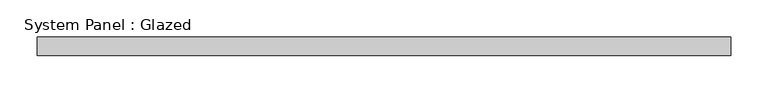
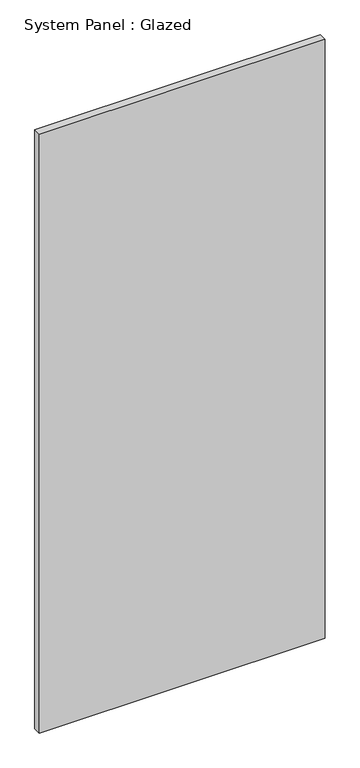
"""IFC4 building model written with IfcOpenShell, lengths in millimetres: plate geometry, System Panel : Glazed."""

import ifcopenshell
import ifcopenshell.guid

model = None  # the IFC model being written
_history = None  # IfcOwnerHistory: only IFC2X3 demands one
_inside = {}  # id of a spatial element -> (the spatial element, [elements in it])
_under = {}  # id of a project, library or spatial element -> (it, [spatial elements below it])
_declared = {}  # id of a project -> (the project, [libraries it declares])
_typed = {}  # id of a type object -> (the type object, [elements of that type])
_made_of = {}  # id of a material, layer set ... -> (it, [elements and type objects made of it])


def new_model(schema):
    """Start an empty IFC model of exactly this schema.

    Asked for "IFC4X3", IfcOpenShell would pick the latest addendum, in which some entities
    have other attributes; the version numbers below select the first issue.
    IFC2X3 requires an IfcOwnerHistory on every rooted entity: one is made here for all.
    """
    global model, _history
    if schema == "IFC4X3":
        model = ifcopenshell.file(schema_version=(4, 3, 0, 0))
    else:
        model = ifcopenshell.file(schema=schema)
    _inside.clear()
    _under.clear()
    _declared.clear()
    _typed.clear()
    _made_of.clear()
    _history = None
    if model.schema == "IFC2X3":
        org = make("IfcOrganization", Name="unknown")
        user = make(
            "IfcPersonAndOrganization",
            ThePerson=make("IfcPerson", FamilyName="unknown"),
            TheOrganization=org,
        )
        app = make(
            "IfcApplication",
            ApplicationDeveloper=org,
            Version="unknown",
            ApplicationFullName="unknown",
            ApplicationIdentifier="unknown",
        )
        _history = make(
            "IfcOwnerHistory",
            OwningUser=user,
            OwningApplication=app,
            ChangeAction="ADDED",
            CreationDate=0,
        )
    return model


def make(cls, **values):
    """One entity of the class cls with the attributes given. An attribute that is None is left unset."""
    return model.create_entity(
        cls, **{name: value for name, value in values.items() if value is not None}
    )


def rooted(cls, **values):
    """An entity with a GlobalId (a new one), such as an element, a storey or a relation."""
    return make(cls, GlobalId=ifcopenshell.guid.new(), OwnerHistory=_history, **values)


def si_unit(unit_type, name, prefix=None):
    """IfcSIUnit, for example si_unit("LENGTHUNIT", "METRE", prefix="MILLI")."""
    return make("IfcSIUnit", UnitType=unit_type, Prefix=prefix, Name=name)


def assignment(units):
    """IfcUnitAssignment: the units of a project."""
    return None if units is None else make("IfcUnitAssignment", Units=units)


def point(xyz):
    """IfcCartesianPoint."""
    return None if xyz is None else make("IfcCartesianPoint", Coordinates=xyz)


def direction(xyz):
    """IfcDirection."""
    return None if xyz is None else make("IfcDirection", DirectionRatios=xyz)


def frame(location, z_axis=None, x_axis=None):
    """IfcAxis2Placement3D, a coordinate frame: its origin and axes. An axis left out is left unset."""
    return make(
        "IfcAxis2Placement3D",
        Location=point(location),
        Axis=direction(z_axis),
        RefDirection=direction(x_axis),
    )


def origin():
    """The frame at (0, 0, 0) with its axes left unset."""
    return frame((0.0, 0.0, 0.0))


def origin_with_axes():
    """The frame at (0, 0, 0) with the z axis (0, 0, 1) and the x axis (1, 0, 0) written out."""
    return frame((0.0, 0.0, 0.0), z_axis=(0.0, 0.0, 1.0), x_axis=(1.0, 0.0, 0.0))


def place(relative_to, where):
    """IfcLocalPlacement: puts the frame where relative to a parent placement (None: the world)."""
    return make(
        "IfcLocalPlacement", PlacementRelTo=relative_to, RelativePlacement=where
    )


def context(
    kind, dimensions, precision=None, world=None, true_north=None, identifier=None
):
    """IfcGeometricRepresentationContext, for example the 3D "Model" context."""
    return make(
        "IfcGeometricRepresentationContext",
        ContextIdentifier=identifier,
        ContextType=kind,
        CoordinateSpaceDimension=dimensions,
        Precision=precision,
        WorldCoordinateSystem=world,
        TrueNorth=true_north,
    )


def project(units=None, contexts=None):
    """IfcProject with its units and contexts."""
    return rooted(
        "IfcProject",
        Name="project",
        RepresentationContexts=contexts,
        UnitsInContext=assignment(units),
    )


def spatial(cls, under=None, at=None, **own):
    """A site, building, storey or space (cls), placed at a placement, below another one or the project."""
    s = rooted(cls, ObjectPlacement=at, **own)
    if under is not None:
        _under.setdefault(under.id(), (under, []))[1].append(s)
    return s


def polyline(points):
    """IfcPolyline through the points."""
    return make("IfcPolyline", Points=[point(p) for p in points])


def outline(outer, holes=None, kind="AREA"):
    """IfcArbitraryClosedProfileDef: a profile drawn as a closed curve; with holes, ...WithVoids."""
    if holes is None:
        return make("IfcArbitraryClosedProfileDef", ProfileType=kind, OuterCurve=outer)
    return make(
        "IfcArbitraryProfileDefWithVoids",
        ProfileType=kind,
        OuterCurve=outer,
        InnerCurves=holes,
    )


def extrude(swept, where, along, depth):
    """IfcExtrudedAreaSolid: the profile swept, set in the frame where, extruded along a direction by depth."""
    return make(
        "IfcExtrudedAreaSolid",
        SweptArea=swept,
        Position=where,
        ExtrudedDirection=direction(along),
        Depth=depth,
    )


def shape(context_of_items, identifier, shape_type, items):
    """IfcShapeRepresentation: the items that make up one representation, for example the "Body"."""
    return make(
        "IfcShapeRepresentation",
        ContextOfItems=context_of_items,
        RepresentationIdentifier=identifier,
        RepresentationType=shape_type,
        Items=items,
    )


def source(mapping_origin, context_of_items, identifier, shape_type, items):
    """IfcRepresentationMap: a shape defined once, which mapped items show again and again."""
    return make(
        "IfcRepresentationMap",
        MappingOrigin=mapping_origin,
        MappedRepresentation=shape(context_of_items, identifier, shape_type, items),
    )


def transform(
    local_origin,
    x_axis=None,
    y_axis=None,
    z_axis=None,
    scale=None,
    scale2=None,
    scale3=None,
    uniform=True,
):
    """IfcCartesianTransformationOperator3D, or its non-uniform kind. x_axis, y_axis, z_axis: its Axis1, 2, 3."""
    if uniform:
        return make(
            "IfcCartesianTransformationOperator3D",
            Axis1=direction(x_axis),
            Axis2=direction(y_axis),
            LocalOrigin=point(local_origin),
            Scale=scale,
            Axis3=direction(z_axis),
        )
    return make(
        "IfcCartesianTransformationOperator3DnonUniform",
        Axis1=direction(x_axis),
        Axis2=direction(y_axis),
        LocalOrigin=point(local_origin),
        Scale=scale,
        Axis3=direction(z_axis),
        Scale2=scale2,
        Scale3=scale3,
    )


def mapped(mapping_source, mapping_target):
    """IfcMappedItem: shows the shape of a source again, moved by a transform."""
    return make(
        "IfcMappedItem", MappingSource=mapping_source, MappingTarget=mapping_target
    )


def made_of(thing, what):
    """Note that an element or type object is made of a material, layer set ...; save() writes the relation."""
    if what is not None:
        _made_of.setdefault(what.id(), (what, []))[1].append(thing)
    return thing


def element(
    cls,
    number,
    at=None,
    inside=None,
    cuts=None,
    type_object=None,
    material=None,
    context=None,
    identifier="Body",
    shape_type=None,
    held_by="IfcProductDefinitionShape",
    body=None,
    shapes=None,
    **own,
):
    """One element of the class cls, such as IfcWall. Its Tag is "e" and its number.

    at: its placement. inside: the storey or other place that contains it. cuts: it is an
    opening in that element (IfcRelVoidsElement). A single representation is given by context,
    identifier, shape_type and body (its items); several are given by shapes. held_by: the class
    of the entity that holds the representations. save() writes the other relations.
    """
    e = rooted(cls, Tag="e%d" % number, ObjectPlacement=at, **own)
    if body is not None:
        shapes = [shape(context, identifier, shape_type, body)]
    if shapes is not None:
        e.Representation = make(held_by, Representations=shapes)
    if inside is not None:
        _inside.setdefault(inside.id(), (inside, []))[1].append(e)
    if cuts is not None:
        rooted(
            "IfcRelVoidsElement", RelatingBuildingElement=cuts, RelatedOpeningElement=e
        )
    if type_object is not None:
        _typed.setdefault(type_object.id(), (type_object, []))[1].append(e)
    return made_of(e, material)


def aggregate(whole, parts):
    """IfcRelAggregates: a whole, such as a stair, and the parts it consists of."""
    return rooted("IfcRelAggregates", RelatingObject=whole, RelatedObjects=parts)


def save(model, path):
    """Write the relations noted so far, then the file.

    IfcRelAggregates (storeys below a building ...), IfcRelContainedInSpatialStructure (elements
    in a storey), IfcRelDefinesByType, IfcRelAssociatesMaterial and IfcRelDeclares: one each for
    every whole, place, type object, material and project.
    """
    for whole, parts in _under.values():
        aggregate(whole, parts)
    for where, things in _inside.values():
        rooted(
            "IfcRelContainedInSpatialStructure",
            RelatedElements=things,
            RelatingStructure=where,
        )
    for kind, things in _typed.values():
        rooted("IfcRelDefinesByType", RelatedObjects=things, RelatingType=kind)
    for what, things in _made_of.values():
        rooted("IfcRelAssociatesMaterial", RelatedObjects=things, RelatingMaterial=what)
    for by, libraries in _declared.values():
        rooted("IfcRelDeclares", RelatingContext=by, RelatedDefinitions=libraries)
    model.write(path)


def system_panel_glazed_4c7b465e(model_context):
    return source(origin(), model_context, "Body", "SweptSolid", [
        extrude(outline(polyline([(467.5, 24.5), (-467.5, 24.5), (-467.5, 49.5), (467.5, 49.5), (467.5, 24.5)])), origin_with_axes(), (0.0, 0.0, 1.0), 2070.0),
    ])


if __name__ == "__main__":
    model = new_model("IFC4")
    model_context = context("Model", 3, world=origin())
    ifc_project = project(units=[si_unit("LENGTHUNIT", "METRE", prefix="MILLI")], contexts=[model_context])
    site = spatial("IfcSite", under=ifc_project)
    building = spatial("IfcBuilding", under=site)
    placement = place(None, origin())
    system_panel_glazed_shape = system_panel_glazed_4c7b465e(model_context)
    element("IfcPlate", 1, ObjectType="System Panel : Glazed", at=placement, inside=building, context=model_context, shape_type="MappedRepresentation", body=[
        mapped(system_panel_glazed_shape, transform((0.0, 0.0, 0.0), x_axis=(1.0, 0.0, 0.0), y_axis=(0.0, 1.0, 0.0), z_axis=(0.0, 0.0, 1.0))),
    ])
    save(model, "model.ifc")

# Revit data of these elements
# Type "System Panel : Glazed"
#   Construction Type Id = "GSP4R"
#   Analytic Construction = "1/8 in Pilkington single glazing"
#   Visual Light Transmittance = 0.9
#   Solar Heat Gain Coefficient = 0.86
#   Heat Transfer Coefficient (U) = 6.7069 W/(m²·K)
#   Define Thermal Properties by = 1
# Element 1 (IfcPlate, "System Panel : Glazed")
#   Materials on its faces: "Glass"
# Materials
#   "Glass": class "Glass", colour RGB 245 245 243, transparency 1, Description = "Soda Lime Glass", Cost = 0
